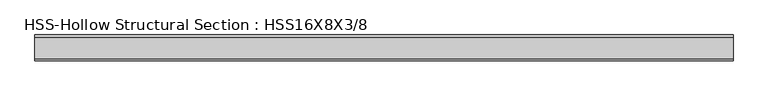
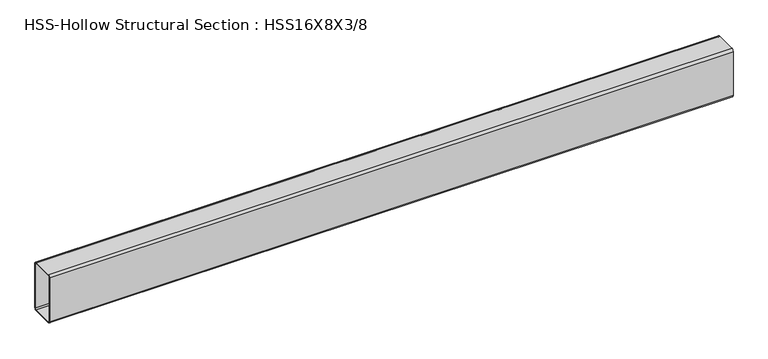
"""IFC4 building model written with IfcOpenShell, lengths in millimetres: beam geometry, HSS-Hollow Structural Section : HSS16X8X3/8."""

from ifc_helpers import new_model, si_unit, point, frame, frame_2d, origin, place, context, project, spatial, polyline, circle_curve, trimmed, segment, composite_curve, outline, extrude, source, transform, mapped, element, save


def hss_hollow_structural_section_hss16x8x3_8_ccc4528a(model_context):
    return source(origin(), model_context, "Body", "SweptSolid", [
        extrude(outline(composite_curve([segment(polyline([(101.6, 185.4708), (101.6, -185.4708)]), True, "CONTINUOUS"), segment(trimmed(circle_curve(frame_2d((83.8708, -185.4708)), 17.7292), [point((101.6, -185.4708))], [point((83.8708, -203.2))], False, "CARTESIAN"), True, "CONTINUOUS"), segment(polyline([(83.8708, -203.2), (-83.8708, -203.2)]), True, "CONTINUOUS"), segment(trimmed(circle_curve(frame_2d((-83.8708, -185.4708)), 17.7292), [point((-83.8708, -203.2))], [point((-101.6, -185.4708))], False, "CARTESIAN"), True, "CONTINUOUS"), segment(polyline([(-101.6, -185.4708), (-101.6, 185.4708)]), True, "CONTINUOUS"), segment(trimmed(circle_curve(frame_2d((-83.8708, 185.4708)), 17.7292), [point((-101.6, 185.4708))], [point((-83.8708, 203.2))], False, "CARTESIAN"), True, "CONTINUOUS"), segment(polyline([(-83.8708, 203.2), (83.8708, 203.2)]), True, "CONTINUOUS"), segment(trimmed(circle_curve(frame_2d((83.8708, 185.4708)), 17.7292), [point((83.8708, 203.2))], [point((101.6, 185.4708))], False, "CARTESIAN"), True, "CONTINUOUS")], self_intersect=False), holes=[composite_curve([segment(trimmed(circle_curve(frame_2d((-83.8708, 185.4708)), 8.8646), [point((-83.8708, 194.3354))], [point((-92.7354, 185.4708))], True, "CARTESIAN"), True, "CONTINUOUS"), segment(polyline([(-92.7354, 185.4708), (-92.7354, -185.4708)]), True, "CONTINUOUS"), segment(trimmed(circle_curve(frame_2d((-83.8708, -185.4708)), 8.8646), [point((-92.7354, -185.4708))], [point((-83.8708, -194.3354))], True, "CARTESIAN"), True, "CONTINUOUS"), segment(polyline([(-83.8708, -194.3354), (83.8708, -194.3354)]), True, "CONTINUOUS"), segment(trimmed(circle_curve(frame_2d((83.8708, -185.4708)), 8.8646), [point((83.8708, -194.3354))], [point((92.7354, -185.4708))], True, "CARTESIAN"), True, "CONTINUOUS"), segment(polyline([(92.7354, -185.4708), (92.7354, 185.4708)]), True, "CONTINUOUS"), segment(trimmed(circle_curve(frame_2d((83.8708, 185.4708)), 8.8646), [point((92.7354, 185.4708))], [point((83.8708, 194.3354))], True, "CARTESIAN"), True, "CONTINUOUS"), segment(polyline([(83.8708, 194.3354), (-83.8708, 194.3354)]), True, "CONTINUOUS")], self_intersect=False)]), frame((-2795.6906869, 0.0, 0.0), z_axis=(1.0, 0.0, 0.0), x_axis=(0.0, 1.0, 0.0)), (0.0, 0.0, 1.0), 5467.8103744),
    ])


if __name__ == "__main__":
    model = new_model("IFC4")
    model_context = context("Model", 3, world=origin())
    ifc_project = project(units=[si_unit("LENGTHUNIT", "METRE", prefix="MILLI")], contexts=[model_context])
    site = spatial("IfcSite", under=ifc_project)
    building = spatial("IfcBuilding", under=site)
    placement = place(None, origin())
    hss_hollow_structural_section_hss16x8x3_8_shape = hss_hollow_structural_section_hss16x8x3_8_ccc4528a(model_context)
    element("IfcBeam", 1, ObjectType="HSS-Hollow Structural Section : HSS16X8X3/8", at=placement, inside=building, context=model_context, shape_type="MappedRepresentation", body=[
        mapped(hss_hollow_structural_section_hss16x8x3_8_shape, transform((0.0, 0.0, 0.0), x_axis=(1.0, 0.0, 0.0), y_axis=(0.0, 1.0, 0.0), z_axis=(0.0, 0.0, 1.0))),
    ])
    save(model, "model.ifc")

# Revit data of these elements
# Type "HSS-Hollow Structural Section : HSS16X8X3/8"
#   Assembly Code = "B10"
#   Shape = "Rect."
#   W = 58.1
#   Ht = 1' - 4"
#   Length [instance default] = 5' - 0"
#   b = 0' - 8"
#   kr = 0' - 0.698"
#   t = 0' - 0.349"
#   A = 0.111111 SF
#   Structural Material [instance default] = Steel ASTM A500, Grade B, Rectangular and Square
# Element 1 (IfcBeam, "HSS-Hollow Structural Section : HSS16X8X3/8")
#   Materials on its faces: "Steel ASTM A500, Grade B, Rectangular and Square"
# Materials
#   "Steel ASTM A500, Grade B, Rectangular and Square": class "Metal", colour RGB 199 199 199, transparency 0, Description = "Carbon steel", Cost = 0
